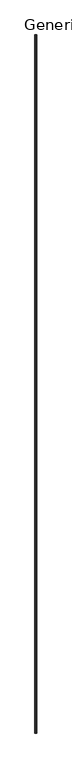
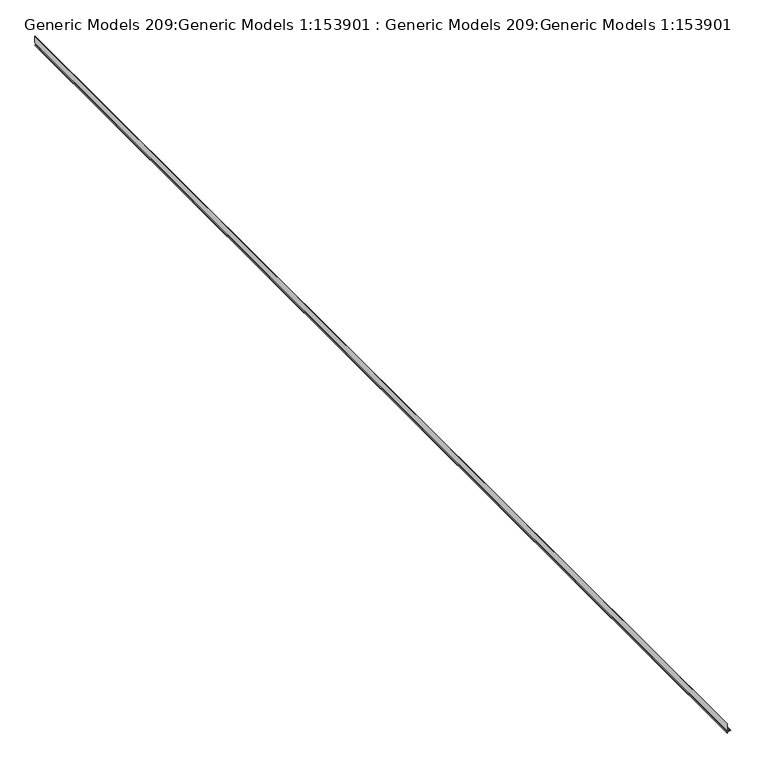
"""IFC4 building model written with IfcOpenShell, lengths in millimetres: proxy geometry, Generic Models 209:Generic Models 1:153901 : Generic Models 209:Generic Models 1:153901."""

from ifc_helpers import new_model, si_unit, frame, origin, place, context, project, spatial, polyline, outline, extrude, source, transform, mapped, element, save


def generic_models_209_generic_models_1_153901_generic_models_861f3ad9(model_context):
    return source(origin(), model_context, "Body", "SweptSolid", [
        extrude(outline(polyline([(3500.3537464, -8201.0597785), (3506.8316945, -8180.9061619), (3513.5672303, -8201.8611619), (3557.6316945, -8201.8611619), (3557.6316945, -8203.1311619), (3512.641451, -8203.1311619), (3506.8316945, -8185.0563642), (3501.3315366, -8202.1679669), (3496.2167862, -8203.1311619), (3495.9817546, -8201.8830994), (3500.3537464, -8201.0597785)])), frame((0.0, -273.9974793, 0.0), z_axis=(0.0, 1.0, 0.0), x_axis=(0.0, 0.0, 1.0)), (0.0, 0.0, 1.0), 7518.4),
    ])


if __name__ == "__main__":
    model = new_model("IFC4")
    model_context = context("Model", 3, world=origin())
    ifc_project = project(units=[si_unit("LENGTHUNIT", "METRE", prefix="MILLI")], contexts=[model_context])
    site = spatial("IfcSite", under=ifc_project)
    building = spatial("IfcBuilding", under=site)
    placement = place(None, origin())
    generic_models_209_generic_models_1_153901_generic_models_shape = generic_models_209_generic_models_1_153901_generic_models_861f3ad9(model_context)
    element("IfcBuildingElementProxy", 1, Name="Generic Models 209:Generic Models 1:153901 : Generic Models 209:Generic Models 1:153901", ObjectType="Generic Models 209:Generic Models 1:153901 : Generic Models 209:Generic Models 1:153901", at=placement, inside=building, context=model_context, shape_type="MappedRepresentation", body=[
        mapped(generic_models_209_generic_models_1_153901_generic_models_shape, transform((0.0, 0.0, 0.0), x_axis=(1.0, 0.0, 0.0), y_axis=(0.0, 1.0, 0.0), z_axis=(0.0, 0.0, 1.0))),
    ])
    save(model, "model.ifc")

# Revit data of these elements
# Type "Generic Models 209:Generic Models 1:153901 : Generic Models 209:Generic Models 1:153901"
#   NameOverride = "Generic Models 209:Generic Models 1:153901"
#   ObjectTypeOverride = "Generic Models 209:Generic Models 1"
#   Reference = "Generic Models 1"
#   Category = "Generic Models"
#   Tag = "153901"
# Element 1 (IfcBuildingElementProxy, "Generic Models 209:Generic Models 1:153901 : Generic Models 209:Generic Models 1:153901")
#   Materials on its faces: "_ 16 GA. COPPER VENTED T REVEAL BEAD (CONT. AROUND PERIMETER OF BEAM) 2987"
# Materials
#   "_ 16 GA. COPPER VENTED T REVEAL BEAD (CONT. AROUND PERIMETER OF BEAM) 2987": class "Unassigned", colour RGB 253 192 103, transparency 0
